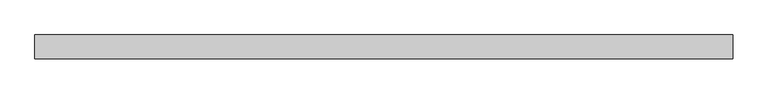
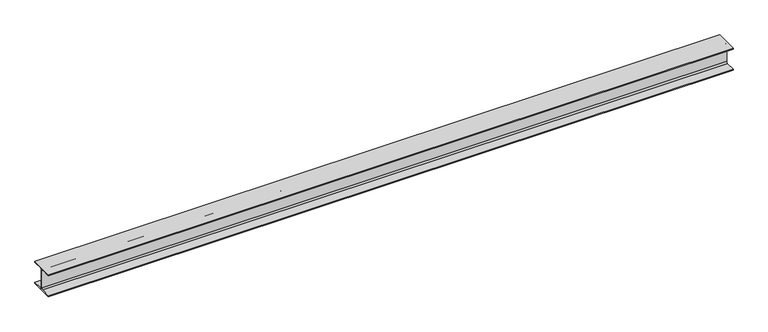
"""IFC4 building model written with IfcOpenShell, lengths in millimetres: beam geometry, 0912_Steel Framing_H-KSD3502 : H_SB_ASB_H-300x300x10x15."""

from ifc_helpers import new_model, si_unit, point, frame, frame_2d, origin, place, context, project, spatial, polyline, circle_curve, trimmed, segment, composite_curve, outline, extrude, source, transform, mapped, element, save


def beam_df7d8c2f(model_context):
    return source(origin(), model_context, "Body", "SweptSolid", [
        extrude(outline(composite_curve([segment(polyline([(150.0, -135.0), (150.0, -150.0), (-150.0, -150.0), (-150.0, -135.0), (-23.0, -135.0)]), True, "CONTINUOUS"), segment(trimmed(circle_curve(frame_2d((-23.0, -117.0)), 18.0), [point((-23.0, -135.0))], [point((-5.0, -117.0))], True, "CARTESIAN"), True, "CONTINUOUS"), segment(polyline([(-5.0, -117.0), (-5.0, 117.0)]), True, "CONTINUOUS"), segment(trimmed(circle_curve(frame_2d((-23.0, 117.0)), 18.0), [point((-5.0, 117.0))], [point((-23.0, 135.0))], True, "CARTESIAN"), True, "CONTINUOUS"), segment(polyline([(-23.0, 135.0), (-150.0, 135.0), (-150.0, 150.0), (150.0, 150.0), (150.0, 135.0), (23.0, 135.0)]), True, "CONTINUOUS"), segment(trimmed(circle_curve(frame_2d((23.0, 117.0)), 18.0), [point((23.0, 135.0))], [point((5.0, 117.0))], True, "CARTESIAN"), True, "CONTINUOUS"), segment(polyline([(5.0, 117.0), (5.0, -117.0)]), True, "CONTINUOUS"), segment(trimmed(circle_curve(frame_2d((23.0, -117.0)), 18.0), [point((5.0, -117.0))], [point((23.0, -135.0))], True, "CARTESIAN"), True, "CONTINUOUS"), segment(polyline([(23.0, -135.0), (150.0, -135.0)]), True, "CONTINUOUS")], self_intersect=False)), frame((-4272.9251782, 0.0, 0.0), z_axis=(1.0, 0.0, 0.0), x_axis=(0.0, 1.0, 0.0)), (0.0, 0.0, 1.0), 8795.3692077),
    ])


if __name__ == "__main__":
    model = new_model("IFC4")
    model_context = context("Model", 3, world=origin())
    ifc_project = project(units=[si_unit("LENGTHUNIT", "METRE", prefix="MILLI")], contexts=[model_context])
    site = spatial("IfcSite", under=ifc_project)
    building = spatial("IfcBuilding", under=site)
    placement = place(None, origin())
    beam_shape = beam_df7d8c2f(model_context)
    element("IfcBeam", 1, ObjectType="0912_Steel Framing_H-KSD3502 : H_SB_ASB_H-300x300x10x15", at=placement, inside=building, context=model_context, shape_type="MappedRepresentation", body=[
        mapped(beam_shape, transform((0.0, 0.0, 0.0), x_axis=(1.0, 0.0, 0.0), y_axis=(0.0, 1.0, 0.0), z_axis=(0.0, 0.0, 1.0))),
    ])
    save(model, "model.ifc")

# Revit data of these elements
# Type "0912_Steel Framing_H-KSD3502 : H_SB_ASB_H-300x300x10x15"
#   H_WM Code_1 = "S01AA001-00001 | Main Steel Structure Fabrication Work | Shelter/Building | Heavy Steel - Standard (Weight≥90KG/M) | Material: (   )"
#   H_WM Code_2 = "S03AA027-00001 | Main Steel Structure Erection Work | Shelter/Building | Heavy Steel (Weight≥90KG/M) | Material: (   )"
#   H_WM Code_3 = "S01AA010-00001 | Main Steel Structure Fabrication Work | Shelter/Building | Steel Painting/Coating | for Non-Fireproofed Steel Surface, Surface Preparation, Primer, Second & Final Coat | Material: (   )"
#   H_Q'ty Cal Type Tag = "SB-Q2"
#   Width = 30.0 cm
#   Web Thickness = 1.0 cm
#   Web Fillet = 1.8 cm
#   Warping Constant = 1370000.0 cm⁶
#   W = 0
#   Torsional Moment of Inertia = 77.00 cm⁴
#   Section Area = 119.8 cm²
#   Plastic Modulus weak axis = 684.0 cm³
#   Plastic Modulus strong axis = 1500.0 cm³
#   Perimeter = 1.75 m²/m
#   Nominal Weight = 94.00 kgf/m
#   Moment of Inertia weak axis = 6750.00 cm⁴
#   Moment of Inertia strong axis = 20400.00 cm⁴
#   Height = 30.0 cm
#   Flange Thickness = 1.5 cm
#   Elastic Modulus weak axis = 450.0 cm³
#   Elastic Modulus strong axis = 1360.0 cm³
#   Centroid Vertical = 15.0 cm
#   Centroid Horizontal = 15.0 cm
#   Ix = 204000000
#   Length [instance default] = 1.5240 m
#   Zx = 1500000
#   b = 0.3000 m
#   h = 0.3000 m
#   r = 0.0180 m
#   s = 0.0100 m
#   t = 0.0150 m
#   A = 0.01198 m²
#   Structural Material [instance default] = Steel, 45-345
#   Assembly Code = ""
# Element 1 (IfcBeam, "0912_Steel Framing_H-KSD3502 : H_SB_ASB_H-300x300x10x15")
#   Structural Material = none
# Materials
#   "Steel, 45-345": class "Metal", colour RGB 189 187 185, transparency 0, Description = "Steel 345 MPa", Cost = 0
